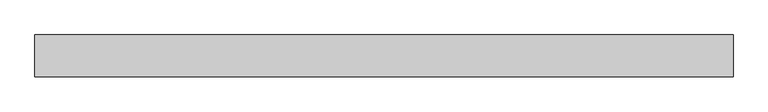
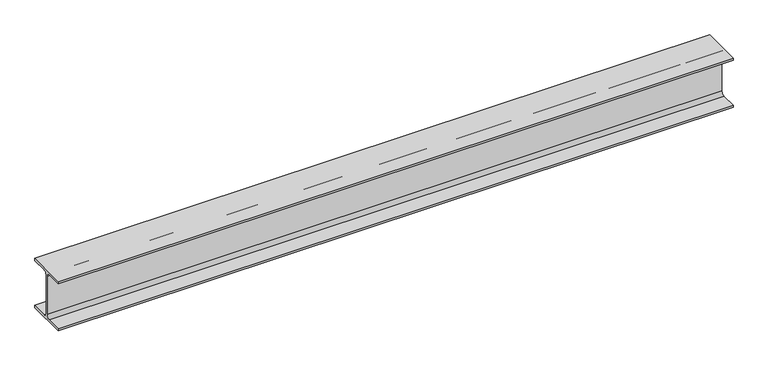
"""IFC4 building model written with IfcOpenShell, lengths in millimetres: beam geometry, 0912_Steel Framing_H-KSD3502 : H_SB_ASB_H-194x150x6x9."""

import ifcopenshell
import ifcopenshell.guid

model = None  # the IFC model being written
_history = None  # IfcOwnerHistory: only IFC2X3 demands one
_inside = {}  # id of a spatial element -> (the spatial element, [elements in it])
_under = {}  # id of a project, library or spatial element -> (it, [spatial elements below it])
_declared = {}  # id of a project -> (the project, [libraries it declares])
_typed = {}  # id of a type object -> (the type object, [elements of that type])
_made_of = {}  # id of a material, layer set ... -> (it, [elements and type objects made of it])


def new_model(schema):
    """Start an empty IFC model of exactly this schema.

    Asked for "IFC4X3", IfcOpenShell would pick the latest addendum, in which some entities
    have other attributes; the version numbers below select the first issue.
    IFC2X3 requires an IfcOwnerHistory on every rooted entity: one is made here for all.
    """
    global model, _history
    if schema == "IFC4X3":
        model = ifcopenshell.file(schema_version=(4, 3, 0, 0))
    else:
        model = ifcopenshell.file(schema=schema)
    _inside.clear()
    _under.clear()
    _declared.clear()
    _typed.clear()
    _made_of.clear()
    _history = None
    if model.schema == "IFC2X3":
        org = make("IfcOrganization", Name="unknown")
        user = make(
            "IfcPersonAndOrganization",
            ThePerson=make("IfcPerson", FamilyName="unknown"),
            TheOrganization=org,
        )
        app = make(
            "IfcApplication",
            ApplicationDeveloper=org,
            Version="unknown",
            ApplicationFullName="unknown",
            ApplicationIdentifier="unknown",
        )
        _history = make(
            "IfcOwnerHistory",
            OwningUser=user,
            OwningApplication=app,
            ChangeAction="ADDED",
            CreationDate=0,
        )
    return model


def make(cls, **values):
    """One entity of the class cls with the attributes given. An attribute that is None is left unset."""
    return model.create_entity(
        cls, **{name: value for name, value in values.items() if value is not None}
    )


def rooted(cls, **values):
    """An entity with a GlobalId (a new one), such as an element, a storey or a relation."""
    return make(cls, GlobalId=ifcopenshell.guid.new(), OwnerHistory=_history, **values)


def si_unit(unit_type, name, prefix=None):
    """IfcSIUnit, for example si_unit("LENGTHUNIT", "METRE", prefix="MILLI")."""
    return make("IfcSIUnit", UnitType=unit_type, Prefix=prefix, Name=name)


def assignment(units):
    """IfcUnitAssignment: the units of a project."""
    return None if units is None else make("IfcUnitAssignment", Units=units)


def point(xyz):
    """IfcCartesianPoint."""
    return None if xyz is None else make("IfcCartesianPoint", Coordinates=xyz)


def direction(xyz):
    """IfcDirection."""
    return None if xyz is None else make("IfcDirection", DirectionRatios=xyz)


def frame(location, z_axis=None, x_axis=None):
    """IfcAxis2Placement3D, a coordinate frame: its origin and axes. An axis left out is left unset."""
    return make(
        "IfcAxis2Placement3D",
        Location=point(location),
        Axis=direction(z_axis),
        RefDirection=direction(x_axis),
    )


def frame_2d(location, x_axis=None):
    """IfcAxis2Placement2D, a coordinate frame in the plane: its origin and x axis."""
    return make(
        "IfcAxis2Placement2D", Location=point(location), RefDirection=direction(x_axis)
    )


def origin():
    """The frame at (0, 0, 0) with its axes left unset."""
    return frame((0.0, 0.0, 0.0))


def place(relative_to, where):
    """IfcLocalPlacement: puts the frame where relative to a parent placement (None: the world)."""
    return make(
        "IfcLocalPlacement", PlacementRelTo=relative_to, RelativePlacement=where
    )


def context(
    kind, dimensions, precision=None, world=None, true_north=None, identifier=None
):
    """IfcGeometricRepresentationContext, for example the 3D "Model" context."""
    return make(
        "IfcGeometricRepresentationContext",
        ContextIdentifier=identifier,
        ContextType=kind,
        CoordinateSpaceDimension=dimensions,
        Precision=precision,
        WorldCoordinateSystem=world,
        TrueNorth=true_north,
    )


def project(units=None, contexts=None):
    """IfcProject with its units and contexts."""
    return rooted(
        "IfcProject",
        Name="project",
        RepresentationContexts=contexts,
        UnitsInContext=assignment(units),
    )


def spatial(cls, under=None, at=None, **own):
    """A site, building, storey or space (cls), placed at a placement, below another one or the project."""
    s = rooted(cls, ObjectPlacement=at, **own)
    if under is not None:
        _under.setdefault(under.id(), (under, []))[1].append(s)
    return s


def polyline(points):
    """IfcPolyline through the points."""
    return make("IfcPolyline", Points=[point(p) for p in points])


def circle_curve(where, radius):
    """IfcCircle in the frame where."""
    return make("IfcCircle", Position=where, Radius=radius)


def trimmed(basis, trim1, trim2, sense, master):
    """IfcTrimmedCurve: the piece of a basis curve between two trims."""
    return make(
        "IfcTrimmedCurve",
        BasisCurve=basis,
        Trim1=trim1,
        Trim2=trim2,
        SenseAgreement=sense,
        MasterRepresentation=master,
    )


def segment(curve, same_sense, transition):
    """IfcCompositeCurveSegment."""
    return make(
        "IfcCompositeCurveSegment",
        Transition=transition,
        SameSense=same_sense,
        ParentCurve=curve,
    )


def composite_curve(segments, self_intersect=None):
    """IfcCompositeCurve: segments joined end to end."""
    return make("IfcCompositeCurve", Segments=segments, SelfIntersect=self_intersect)


def outline(outer, holes=None, kind="AREA"):
    """IfcArbitraryClosedProfileDef: a profile drawn as a closed curve; with holes, ...WithVoids."""
    if holes is None:
        return make("IfcArbitraryClosedProfileDef", ProfileType=kind, OuterCurve=outer)
    return make(
        "IfcArbitraryProfileDefWithVoids",
        ProfileType=kind,
        OuterCurve=outer,
        InnerCurves=holes,
    )


def extrude(swept, where, along, depth):
    """IfcExtrudedAreaSolid: the profile swept, set in the frame where, extruded along a direction by depth."""
    return make(
        "IfcExtrudedAreaSolid",
        SweptArea=swept,
        Position=where,
        ExtrudedDirection=direction(along),
        Depth=depth,
    )


def shape(context_of_items, identifier, shape_type, items):
    """IfcShapeRepresentation: the items that make up one representation, for example the "Body"."""
    return make(
        "IfcShapeRepresentation",
        ContextOfItems=context_of_items,
        RepresentationIdentifier=identifier,
        RepresentationType=shape_type,
        Items=items,
    )


def source(mapping_origin, context_of_items, identifier, shape_type, items):
    """IfcRepresentationMap: a shape defined once, which mapped items show again and again."""
    return make(
        "IfcRepresentationMap",
        MappingOrigin=mapping_origin,
        MappedRepresentation=shape(context_of_items, identifier, shape_type, items),
    )


def transform(
    local_origin,
    x_axis=None,
    y_axis=None,
    z_axis=None,
    scale=None,
    scale2=None,
    scale3=None,
    uniform=True,
):
    """IfcCartesianTransformationOperator3D, or its non-uniform kind. x_axis, y_axis, z_axis: its Axis1, 2, 3."""
    if uniform:
        return make(
            "IfcCartesianTransformationOperator3D",
            Axis1=direction(x_axis),
            Axis2=direction(y_axis),
            LocalOrigin=point(local_origin),
            Scale=scale,
            Axis3=direction(z_axis),
        )
    return make(
        "IfcCartesianTransformationOperator3DnonUniform",
        Axis1=direction(x_axis),
        Axis2=direction(y_axis),
        LocalOrigin=point(local_origin),
        Scale=scale,
        Axis3=direction(z_axis),
        Scale2=scale2,
        Scale3=scale3,
    )


def mapped(mapping_source, mapping_target):
    """IfcMappedItem: shows the shape of a source again, moved by a transform."""
    return make(
        "IfcMappedItem", MappingSource=mapping_source, MappingTarget=mapping_target
    )


def made_of(thing, what):
    """Note that an element or type object is made of a material, layer set ...; save() writes the relation."""
    if what is not None:
        _made_of.setdefault(what.id(), (what, []))[1].append(thing)
    return thing


def element(
    cls,
    number,
    at=None,
    inside=None,
    cuts=None,
    type_object=None,
    material=None,
    context=None,
    identifier="Body",
    shape_type=None,
    held_by="IfcProductDefinitionShape",
    body=None,
    shapes=None,
    **own,
):
    """One element of the class cls, such as IfcWall. Its Tag is "e" and its number.

    at: its placement. inside: the storey or other place that contains it. cuts: it is an
    opening in that element (IfcRelVoidsElement). A single representation is given by context,
    identifier, shape_type and body (its items); several are given by shapes. held_by: the class
    of the entity that holds the representations. save() writes the other relations.
    """
    e = rooted(cls, Tag="e%d" % number, ObjectPlacement=at, **own)
    if body is not None:
        shapes = [shape(context, identifier, shape_type, body)]
    if shapes is not None:
        e.Representation = make(held_by, Representations=shapes)
    if inside is not None:
        _inside.setdefault(inside.id(), (inside, []))[1].append(e)
    if cuts is not None:
        rooted(
            "IfcRelVoidsElement", RelatingBuildingElement=cuts, RelatedOpeningElement=e
        )
    if type_object is not None:
        _typed.setdefault(type_object.id(), (type_object, []))[1].append(e)
    return made_of(e, material)


def aggregate(whole, parts):
    """IfcRelAggregates: a whole, such as a stair, and the parts it consists of."""
    return rooted("IfcRelAggregates", RelatingObject=whole, RelatedObjects=parts)


def save(model, path):
    """Write the relations noted so far, then the file.

    IfcRelAggregates (storeys below a building ...), IfcRelContainedInSpatialStructure (elements
    in a storey), IfcRelDefinesByType, IfcRelAssociatesMaterial and IfcRelDeclares: one each for
    every whole, place, type object, material and project.
    """
    for whole, parts in _under.values():
        aggregate(whole, parts)
    for where, things in _inside.values():
        rooted(
            "IfcRelContainedInSpatialStructure",
            RelatedElements=things,
            RelatingStructure=where,
        )
    for kind, things in _typed.values():
        rooted("IfcRelDefinesByType", RelatedObjects=things, RelatingType=kind)
    for what, things in _made_of.values():
        rooted("IfcRelAssociatesMaterial", RelatedObjects=things, RelatingMaterial=what)
    for by, libraries in _declared.values():
        rooted("IfcRelDeclares", RelatingContext=by, RelatedDefinitions=libraries)
    model.write(path)


def beam_24c894de(model_context):
    return source(origin(), model_context, "Body", "SweptSolid", [
        extrude(outline(composite_curve([segment(polyline([(75.0, -88.0), (75.0, -97.0), (-75.0, -97.0), (-75.0, -88.0), (-16.0, -88.0)]), True, "CONTINUOUS"), segment(trimmed(circle_curve(frame_2d((-16.0, -75.0)), 13.0), [point((-16.0, -88.0))], [point((-3.0, -75.0))], True, "CARTESIAN"), True, "CONTINUOUS"), segment(polyline([(-3.0, -75.0), (-3.0, 75.0)]), True, "CONTINUOUS"), segment(trimmed(circle_curve(frame_2d((-16.0, 75.0)), 13.0), [point((-3.0, 75.0))], [point((-16.0, 88.0))], True, "CARTESIAN"), True, "CONTINUOUS"), segment(polyline([(-16.0, 88.0), (-75.0, 88.0), (-75.0, 97.0), (75.0, 97.0), (75.0, 88.0), (16.0, 88.0)]), True, "CONTINUOUS"), segment(trimmed(circle_curve(frame_2d((16.0, 75.0)), 13.0), [point((16.0, 88.0))], [point((3.0, 75.0))], True, "CARTESIAN"), True, "CONTINUOUS"), segment(polyline([(3.0, 75.0), (3.0, -75.0)]), True, "CONTINUOUS"), segment(trimmed(circle_curve(frame_2d((16.0, -75.0)), 13.0), [point((3.0, -75.0))], [point((16.0, -88.0))], True, "CARTESIAN"), True, "CONTINUOUS"), segment(polyline([(16.0, -88.0), (75.0, -88.0)]), True, "CONTINUOUS")], self_intersect=False)), frame((-1253.7727018, 0.0, 0.0), z_axis=(1.0, 0.0, 0.0), x_axis=(0.0, 1.0, 0.0)), (0.0, 0.0, 1.0), 2507.5454036),
    ])


if __name__ == "__main__":
    model = new_model("IFC4")
    model_context = context("Model", 3, world=origin())
    ifc_project = project(units=[si_unit("LENGTHUNIT", "METRE", prefix="MILLI")], contexts=[model_context])
    site = spatial("IfcSite", under=ifc_project)
    building = spatial("IfcBuilding", under=site)
    placement = place(None, origin())
    beam_shape = beam_24c894de(model_context)
    element("IfcBeam", 1, ObjectType="0912_Steel Framing_H-KSD3502 : H_SB_ASB_H-194x150x6x9", at=placement, inside=building, context=model_context, shape_type="MappedRepresentation", body=[
        mapped(beam_shape, transform((0.0, 0.0, 0.0), x_axis=(1.0, 0.0, 0.0), y_axis=(0.0, 1.0, 0.0), z_axis=(0.0, 0.0, 1.0))),
    ])
    save(model, "model.ifc")

# Revit data of these elements
# Type "0912_Steel Framing_H-KSD3502 : H_SB_ASB_H-194x150x6x9"
#   H_WM Code_1 = "S01AA002-00001 | Main Steel Structure Fabrication Work | Shelter/Building | Medium Steel - Standard (90KG/M>Weight≥30KG/M) | Material: (   )"
#   H_WM Code_2 = "S03AA028-00001 | Main Steel Structure Erection Work | Shelter/Building | Medium Steel (90KG/M>Weight≥30KG/M) | Material: (   )"
#   H_WM Code_3 = "S01AA010-00001 | Main Steel Structure Fabrication Work | Shelter/Building | Steel Painting/Coating | for Non-Fireproofed Steel Surface, Surface Preparation, Primer, Second & Final Coat | Material: (   )"
#   H_Q'ty Cal Type Tag = "SB-Q2"
#   Width = 15.0 cm
#   Web Thickness = 0.6 cm
#   Web Fillet = 1.3 cm
#   Warping Constant = 43316.0 cm⁶
#   W = 0
#   Torsional Moment of Inertia = 8.622 cm⁴
#   Section Area = 39.01 cm²
#   Plastic Modulus weak axis = 104.0 cm³
#   Plastic Modulus strong axis = 309.0 cm³
#   Perimeter = 0.95 m²/m
#   Nominal Weight = 30.60 kgf/m
#   Moment of Inertia weak axis = 507.00 cm⁴
#   Moment of Inertia strong axis = 2690.00 cm⁴
#   Height = 19.4 cm
#   Flange Thickness = 0.9 cm
#   Elastic Modulus weak axis = 67.6 cm³
#   Elastic Modulus strong axis = 277.0 cm³
#   Centroid Vertical = 9.7 cm
#   Centroid Horizontal = 7.5 cm
#   Ix = 26900000
#   Length [instance default] = 1.5240 m
#   Zx = 309000
#   b = 0.1500 m
#   h = 0.1940 m
#   r = 0.0130 m
#   s = 0.0060 m
#   t = 0.0090 m
#   A = 0.003901 m²
#   Structural Material [instance default] = Steel, 45-345
#   Assembly Code = ""
# Element 1 (IfcBeam, "0912_Steel Framing_H-KSD3502 : H_SB_ASB_H-194x150x6x9")
#   Structural Material = none
# Materials
#   "Steel, 45-345": class "Metal", colour RGB 189 187 185, transparency 0, Description = "Steel 345 MPa", Cost = 0
